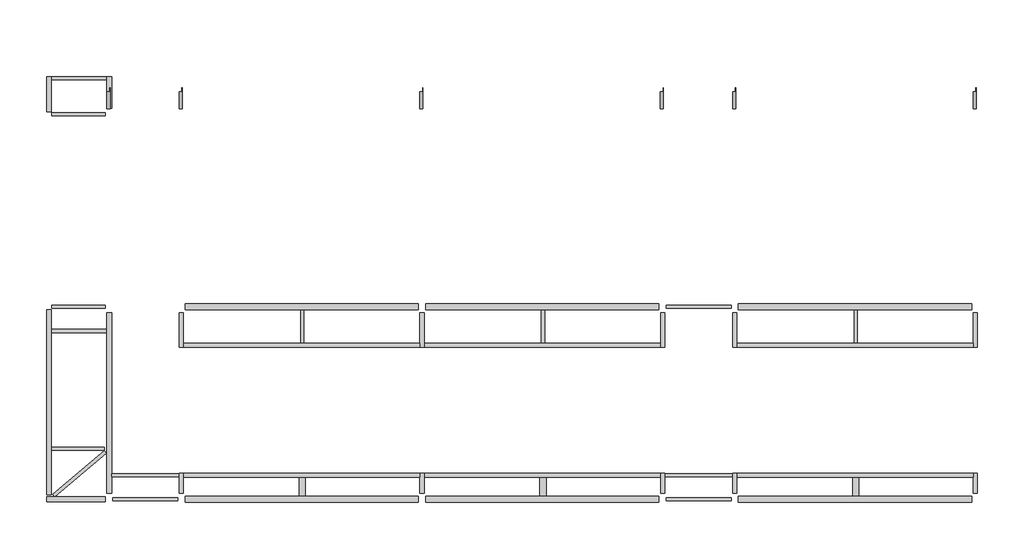
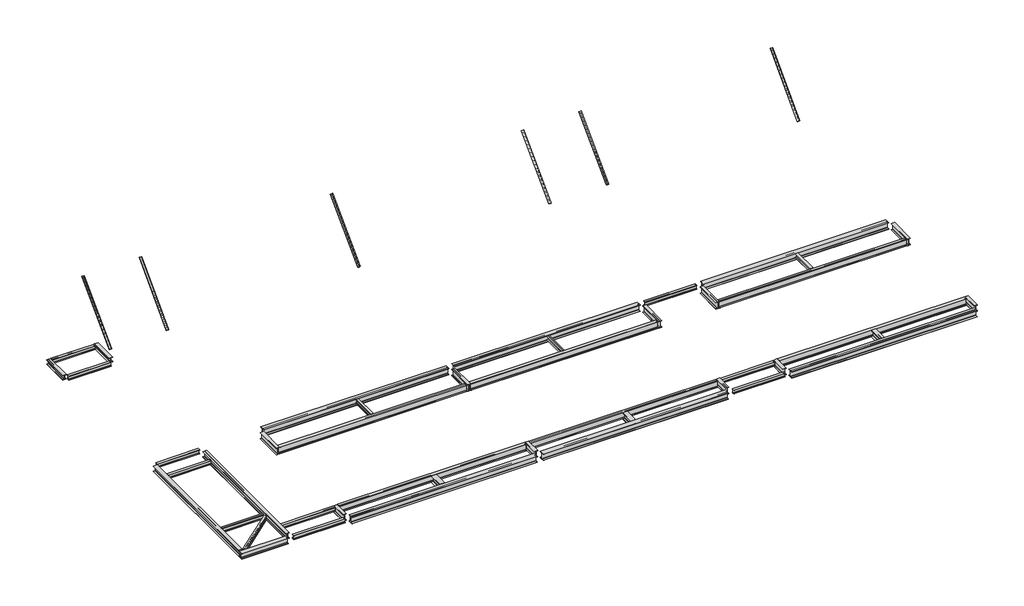
# One storey: 50 beams.
"""IFC4 building model written with IfcOpenShell, lengths in millimetres."""

import ifcopenshell
import ifcopenshell.guid

model = None  # the IFC model being written
_history = None  # IfcOwnerHistory: only IFC2X3 demands one
_inside = {}  # id of a spatial element -> (the spatial element, [elements in it])
_under = {}  # id of a project, library or spatial element -> (it, [spatial elements below it])
_declared = {}  # id of a project -> (the project, [libraries it declares])
_typed = {}  # id of a type object -> (the type object, [elements of that type])
_made_of = {}  # id of a material, layer set ... -> (it, [elements and type objects made of it])


def new_model(schema):
    """Start an empty IFC model of exactly this schema.

    Asked for "IFC4X3", IfcOpenShell would pick the latest addendum, in which some entities
    have other attributes; the version numbers below select the first issue.
    IFC2X3 requires an IfcOwnerHistory on every rooted entity: one is made here for all.
    """
    global model, _history
    if schema == "IFC4X3":
        model = ifcopenshell.file(schema_version=(4, 3, 0, 0))
    else:
        model = ifcopenshell.file(schema=schema)
    _inside.clear()
    _under.clear()
    _declared.clear()
    _typed.clear()
    _made_of.clear()
    _history = None
    if model.schema == "IFC2X3":
        org = make("IfcOrganization", Name="unknown")
        user = make(
            "IfcPersonAndOrganization",
            ThePerson=make("IfcPerson", FamilyName="unknown"),
            TheOrganization=org,
        )
        app = make(
            "IfcApplication",
            ApplicationDeveloper=org,
            Version="unknown",
            ApplicationFullName="unknown",
            ApplicationIdentifier="unknown",
        )
        _history = make(
            "IfcOwnerHistory",
            OwningUser=user,
            OwningApplication=app,
            ChangeAction="ADDED",
            CreationDate=0,
        )
    return model


def make(cls, **values):
    """One entity of the class cls with the attributes given. An attribute that is None is left unset."""
    return model.create_entity(
        cls, **{name: value for name, value in values.items() if value is not None}
    )


def rooted(cls, **values):
    """An entity with a GlobalId (a new one), such as an element, a storey or a relation."""
    return make(cls, GlobalId=ifcopenshell.guid.new(), OwnerHistory=_history, **values)


def si_unit(unit_type, name, prefix=None):
    """IfcSIUnit, for example si_unit("LENGTHUNIT", "METRE", prefix="MILLI")."""
    return make("IfcSIUnit", UnitType=unit_type, Prefix=prefix, Name=name)


def assignment(units):
    """IfcUnitAssignment: the units of a project."""
    return None if units is None else make("IfcUnitAssignment", Units=units)


def point(xyz):
    """IfcCartesianPoint."""
    return None if xyz is None else make("IfcCartesianPoint", Coordinates=xyz)


def direction(xyz):
    """IfcDirection."""
    return None if xyz is None else make("IfcDirection", DirectionRatios=xyz)


def frame(location, z_axis=None, x_axis=None):
    """IfcAxis2Placement3D, a coordinate frame: its origin and axes. An axis left out is left unset."""
    return make(
        "IfcAxis2Placement3D",
        Location=point(location),
        Axis=direction(z_axis),
        RefDirection=direction(x_axis),
    )


def frame_2d(location, x_axis=None):
    """IfcAxis2Placement2D, a coordinate frame in the plane: its origin and x axis."""
    return make(
        "IfcAxis2Placement2D", Location=point(location), RefDirection=direction(x_axis)
    )


def origin():
    """The frame at (0, 0, 0) with its axes left unset."""
    return frame((0.0, 0.0, 0.0))


def place(relative_to, where):
    """IfcLocalPlacement: puts the frame where relative to a parent placement (None: the world)."""
    return make(
        "IfcLocalPlacement", PlacementRelTo=relative_to, RelativePlacement=where
    )


def context(
    kind, dimensions, precision=None, world=None, true_north=None, identifier=None
):
    """IfcGeometricRepresentationContext, for example the 3D "Model" context."""
    return make(
        "IfcGeometricRepresentationContext",
        ContextIdentifier=identifier,
        ContextType=kind,
        CoordinateSpaceDimension=dimensions,
        Precision=precision,
        WorldCoordinateSystem=world,
        TrueNorth=true_north,
    )


def project(units=None, contexts=None):
    """IfcProject with its units and contexts."""
    return rooted(
        "IfcProject",
        Name="project",
        RepresentationContexts=contexts,
        UnitsInContext=assignment(units),
    )


def spatial(cls, under=None, at=None, **own):
    """A site, building, storey or space (cls), placed at a placement, below another one or the project."""
    s = rooted(cls, ObjectPlacement=at, **own)
    if under is not None:
        _under.setdefault(under.id(), (under, []))[1].append(s)
    return s


def polyline(points):
    """IfcPolyline through the points."""
    return make("IfcPolyline", Points=[point(p) for p in points])


def circle_curve(where, radius):
    """IfcCircle in the frame where."""
    return make("IfcCircle", Position=where, Radius=radius)


def trimmed(basis, trim1, trim2, sense, master):
    """IfcTrimmedCurve: the piece of a basis curve between two trims."""
    return make(
        "IfcTrimmedCurve",
        BasisCurve=basis,
        Trim1=trim1,
        Trim2=trim2,
        SenseAgreement=sense,
        MasterRepresentation=master,
    )


def segment(curve, same_sense, transition):
    """IfcCompositeCurveSegment."""
    return make(
        "IfcCompositeCurveSegment",
        Transition=transition,
        SameSense=same_sense,
        ParentCurve=curve,
    )


def composite_curve(segments, self_intersect=None):
    """IfcCompositeCurve: segments joined end to end."""
    return make("IfcCompositeCurve", Segments=segments, SelfIntersect=self_intersect)


def outline(outer, holes=None, kind="AREA"):
    """IfcArbitraryClosedProfileDef: a profile drawn as a closed curve; with holes, ...WithVoids."""
    if holes is None:
        return make("IfcArbitraryClosedProfileDef", ProfileType=kind, OuterCurve=outer)
    return make(
        "IfcArbitraryProfileDefWithVoids",
        ProfileType=kind,
        OuterCurve=outer,
        InnerCurves=holes,
    )


def extrude(swept, where, along, depth):
    """IfcExtrudedAreaSolid: the profile swept, set in the frame where, extruded along a direction by depth."""
    return make(
        "IfcExtrudedAreaSolid",
        SweptArea=swept,
        Position=where,
        ExtrudedDirection=direction(along),
        Depth=depth,
    )


def shape(context_of_items, identifier, shape_type, items):
    """IfcShapeRepresentation: the items that make up one representation, for example the "Body"."""
    return make(
        "IfcShapeRepresentation",
        ContextOfItems=context_of_items,
        RepresentationIdentifier=identifier,
        RepresentationType=shape_type,
        Items=items,
    )


def source(mapping_origin, context_of_items, identifier, shape_type, items):
    """IfcRepresentationMap: a shape defined once, which mapped items show again and again."""
    return make(
        "IfcRepresentationMap",
        MappingOrigin=mapping_origin,
        MappedRepresentation=shape(context_of_items, identifier, shape_type, items),
    )


def transform(
    local_origin,
    x_axis=None,
    y_axis=None,
    z_axis=None,
    scale=None,
    scale2=None,
    scale3=None,
    uniform=True,
):
    """IfcCartesianTransformationOperator3D, or its non-uniform kind. x_axis, y_axis, z_axis: its Axis1, 2, 3."""
    if uniform:
        return make(
            "IfcCartesianTransformationOperator3D",
            Axis1=direction(x_axis),
            Axis2=direction(y_axis),
            LocalOrigin=point(local_origin),
            Scale=scale,
            Axis3=direction(z_axis),
        )
    return make(
        "IfcCartesianTransformationOperator3DnonUniform",
        Axis1=direction(x_axis),
        Axis2=direction(y_axis),
        LocalOrigin=point(local_origin),
        Scale=scale,
        Axis3=direction(z_axis),
        Scale2=scale2,
        Scale3=scale3,
    )


def mapped(mapping_source, mapping_target):
    """IfcMappedItem: shows the shape of a source again, moved by a transform."""
    return make(
        "IfcMappedItem", MappingSource=mapping_source, MappingTarget=mapping_target
    )


def made_of(thing, what):
    """Note that an element or type object is made of a material, layer set ...; save() writes the relation."""
    if what is not None:
        _made_of.setdefault(what.id(), (what, []))[1].append(thing)
    return thing


def element(
    cls,
    number,
    at=None,
    inside=None,
    cuts=None,
    type_object=None,
    material=None,
    context=None,
    identifier="Body",
    shape_type=None,
    held_by="IfcProductDefinitionShape",
    body=None,
    shapes=None,
    **own,
):
    """One element of the class cls, such as IfcWall. Its Tag is "e" and its number.

    at: its placement. inside: the storey or other place that contains it. cuts: it is an
    opening in that element (IfcRelVoidsElement). A single representation is given by context,
    identifier, shape_type and body (its items); several are given by shapes. held_by: the class
    of the entity that holds the representations. save() writes the other relations.
    """
    e = rooted(cls, Tag="e%d" % number, ObjectPlacement=at, **own)
    if body is not None:
        shapes = [shape(context, identifier, shape_type, body)]
    if shapes is not None:
        e.Representation = make(held_by, Representations=shapes)
    if inside is not None:
        _inside.setdefault(inside.id(), (inside, []))[1].append(e)
    if cuts is not None:
        rooted(
            "IfcRelVoidsElement", RelatingBuildingElement=cuts, RelatedOpeningElement=e
        )
    if type_object is not None:
        _typed.setdefault(type_object.id(), (type_object, []))[1].append(e)
    return made_of(e, material)


def aggregate(whole, parts):
    """IfcRelAggregates: a whole, such as a stair, and the parts it consists of."""
    return rooted("IfcRelAggregates", RelatingObject=whole, RelatedObjects=parts)


def save(model, path):
    """Write the relations noted so far, then the file.

    IfcRelAggregates (storeys below a building ...), IfcRelContainedInSpatialStructure (elements
    in a storey), IfcRelDefinesByType, IfcRelAssociatesMaterial and IfcRelDeclares: one each for
    every whole, place, type object, material and project.
    """
    for whole, parts in _under.values():
        aggregate(whole, parts)
    for where, things in _inside.values():
        rooted(
            "IfcRelContainedInSpatialStructure",
            RelatedElements=things,
            RelatingStructure=where,
        )
    for kind, things in _typed.values():
        rooted("IfcRelDefinesByType", RelatedObjects=things, RelatingType=kind)
    for what, things in _made_of.values():
        rooted("IfcRelAssociatesMaterial", RelatedObjects=things, RelatingMaterial=what)
    for by, libraries in _declared.values():
        rooted("IfcRelDeclares", RelatingContext=by, RelatedDefinitions=libraries)
    model.write(path)


def beam_14297e1c(model_context):
    return source(origin(), model_context, "Body", "SweptSolid", [
        extrude(outline(composite_curve([segment(polyline([(36.4, 36.4), (36.4, -93.6)]), True, "CONTINUOUS"), segment(trimmed(circle_curve(frame_2d((36.4, -81.6)), 12.0), [point((36.4, -93.6))], [point((24.4, -81.6))], False, "CARTESIAN"), True, "CONTINUOUS"), segment(polyline([(24.4, -81.6), (24.4, 12.4)]), True, "CONTINUOUS"), segment(trimmed(circle_curve(frame_2d((12.4, 12.4)), 12.0), [point((24.4, 12.4))], [point((12.4, 24.4))], True, "CARTESIAN"), True, "CONTINUOUS"), segment(polyline([(12.4, 24.4), (-81.6, 24.4)]), True, "CONTINUOUS"), segment(trimmed(circle_curve(frame_2d((-81.6, 36.4)), 12.0), [point((-81.6, 24.4))], [point((-93.6, 36.4))], False, "CARTESIAN"), True, "CONTINUOUS"), segment(polyline([(-93.6, 36.4), (36.4, 36.4)]), True, "CONTINUOUS")], self_intersect=False)), frame((-1819.863551, 0.0, 0.0), z_axis=(1.0, 0.0, 0.0), x_axis=(0.0, 1.0, 0.0)), (0.0, 0.0, 1.0), 3551.9244278),
    ])


def steel_framing_w_astm_a6m_f33feb28(model_context):
    return source(origin(), model_context, "Body", "SweptSolid", [
        extrude(outline(composite_curve([segment(polyline([(67.0, -94.8), (67.0, -105.0), (-67.0, -105.0), (-67.0, -94.8), (-10.775, -94.8)]), True, "CONTINUOUS"), segment(trimmed(circle_curve(frame_2d((-10.775, -87.2)), 7.6), [point((-10.775, -94.8))], [point((-3.175, -87.2))], True, "CARTESIAN"), True, "CONTINUOUS"), segment(polyline([(-3.175, -87.2), (-3.175, 87.2)]), True, "CONTINUOUS"), segment(trimmed(circle_curve(frame_2d((-10.775, 87.2)), 7.6), [point((-3.175, 87.2))], [point((-10.775, 94.8))], True, "CARTESIAN"), True, "CONTINUOUS"), segment(polyline([(-10.775, 94.8), (-67.0, 94.8), (-67.0, 105.0), (67.0, 105.0), (67.0, 94.8), (10.775, 94.8)]), True, "CONTINUOUS"), segment(trimmed(circle_curve(frame_2d((10.775, 87.2)), 7.6), [point((10.775, 94.8))], [point((3.175, 87.2))], True, "CARTESIAN"), True, "CONTINUOUS"), segment(polyline([(3.175, 87.2), (3.175, -87.2)]), True, "CONTINUOUS"), segment(trimmed(circle_curve(frame_2d((10.775, -87.2)), 7.6), [point((3.175, -87.2))], [point((10.775, -94.8))], True, "CARTESIAN"), True, "CONTINUOUS"), segment(polyline([(10.775, -94.8), (67.0, -94.8)]), True, "CONTINUOUS")], self_intersect=False)), frame((-1346.3, 0.0, 0.0), z_axis=(1.0, 0.0, 0.0), x_axis=(0.0, 1.0, 0.0)), (0.0, 0.0, 1.0), 2692.6),
    ])


def steel_framing_w_astm_a6m_9ad7bea0(model_context):
    return source(origin(), model_context, "Body", "SweptSolid", [
        extrude(outline(composite_curve([segment(polyline([(67.0, -94.8), (67.0, -105.0), (-67.0, -105.0), (-67.0, -94.8), (-10.775, -94.8)]), True, "CONTINUOUS"), segment(trimmed(circle_curve(frame_2d((-10.775, -87.2)), 7.6), [point((-10.775, -94.8))], [point((-3.175, -87.2))], True, "CARTESIAN"), True, "CONTINUOUS"), segment(polyline([(-3.175, -87.2), (-3.175, 87.2)]), True, "CONTINUOUS"), segment(trimmed(circle_curve(frame_2d((-10.775, 87.2)), 7.6), [point((-3.175, 87.2))], [point((-10.775, 94.8))], True, "CARTESIAN"), True, "CONTINUOUS"), segment(polyline([(-10.775, 94.8), (-67.0, 94.8), (-67.0, 105.0), (67.0, 105.0), (67.0, 94.8), (10.775, 94.8)]), True, "CONTINUOUS"), segment(trimmed(circle_curve(frame_2d((10.775, 87.2)), 7.6), [point((10.775, 94.8))], [point((3.175, 87.2))], True, "CARTESIAN"), True, "CONTINUOUS"), segment(polyline([(3.175, 87.2), (3.175, -87.2)]), True, "CONTINUOUS"), segment(trimmed(circle_curve(frame_2d((10.775, -87.2)), 7.6), [point((3.175, -87.2))], [point((10.775, -94.8))], True, "CARTESIAN"), True, "CONTINUOUS"), segment(polyline([(10.775, -94.8), (67.0, -94.8)]), True, "CONTINUOUS")], self_intersect=False)), frame((-1135.3, 0.0, 0.0), z_axis=(1.0, 0.0, 0.0), x_axis=(0.0, 1.0, 0.0)), (0.0, 0.0, 1.0), 2231.6),
    ])


def steel_framing_w_astm_a6m_5f95f2a9(model_context):
    return source(origin(), model_context, "Body", "SweptSolid", [
        extrude(outline(composite_curve([segment(polyline([(67.0, -94.8), (67.0, -105.0), (-67.0, -105.0), (-67.0, -94.8), (-10.775, -94.8)]), True, "CONTINUOUS"), segment(trimmed(circle_curve(frame_2d((-10.775, -87.2)), 7.6), [point((-10.775, -94.8))], [point((-3.175, -87.2))], True, "CARTESIAN"), True, "CONTINUOUS"), segment(polyline([(-3.175, -87.2), (-3.175, 87.2)]), True, "CONTINUOUS"), segment(trimmed(circle_curve(frame_2d((-10.775, 87.2)), 7.6), [point((-3.175, 87.2))], [point((-10.775, 94.8))], True, "CARTESIAN"), True, "CONTINUOUS"), segment(polyline([(-10.775, 94.8), (-67.0, 94.8), (-67.0, 105.0), (67.0, 105.0), (67.0, 94.8), (10.775, 94.8)]), True, "CONTINUOUS"), segment(trimmed(circle_curve(frame_2d((10.775, 87.2)), 7.6), [point((10.775, 94.8))], [point((3.175, 87.2))], True, "CARTESIAN"), True, "CONTINUOUS"), segment(polyline([(3.175, 87.2), (3.175, -87.2)]), True, "CONTINUOUS"), segment(trimmed(circle_curve(frame_2d((10.775, -87.2)), 7.6), [point((3.175, -87.2))], [point((10.775, -94.8))], True, "CARTESIAN"), True, "CONTINUOUS"), segment(polyline([(10.775, -94.8), (67.0, -94.8)]), True, "CONTINUOUS")], self_intersect=False)), frame((-1401.8, 0.0, 0.0), z_axis=(1.0, 0.0, 0.0), x_axis=(0.0, 1.0, 0.0)), (0.0, 0.0, 1.0), 2803.6),
    ])


def steel_framing_w_astm_a6m_17837fc5(model_context):
    return source(origin(), model_context, "Body", "SweptSolid", [
        extrude(outline(composite_curve([segment(polyline([(127.0, -160.1), (127.0, -176.5), (-127.0, -176.5), (-127.0, -160.1), (-19.865, -160.1)]), True, "CONTINUOUS"), segment(trimmed(circle_curve(frame_2d((-19.865, -145.0)), 15.1), [point((-19.865, -160.1))], [point((-4.765, -145.0))], True, "CARTESIAN"), True, "CONTINUOUS"), segment(polyline([(-4.765, -145.0), (-4.765, 145.0)]), True, "CONTINUOUS"), segment(trimmed(circle_curve(frame_2d((-19.865, 145.0)), 15.1), [point((-4.765, 145.0))], [point((-19.865, 160.1))], True, "CARTESIAN"), True, "CONTINUOUS"), segment(polyline([(-19.865, 160.1), (-127.0, 160.1), (-127.0, 176.5), (127.0, 176.5), (127.0, 160.1), (19.865, 160.1)]), True, "CONTINUOUS"), segment(trimmed(circle_curve(frame_2d((19.865, 145.0)), 15.1), [point((19.865, 160.1))], [point((4.765, 145.0))], True, "CARTESIAN"), True, "CONTINUOUS"), segment(polyline([(4.765, 145.0), (4.765, -145.0)]), True, "CONTINUOUS"), segment(trimmed(circle_curve(frame_2d((19.865, -145.0)), 15.1), [point((4.765, -145.0))], [point((19.865, -160.1))], True, "CARTESIAN"), True, "CONTINUOUS"), segment(polyline([(19.865, -160.1), (127.0, -160.1)]), True, "CONTINUOUS")], self_intersect=False)), frame((-4846.3, 0.0, 0.0), z_axis=(1.0, 0.0, 0.0), x_axis=(0.0, 1.0, 0.0)), (0.0, 0.0, 1.0), 9692.6),
    ])


def steel_framing_w_astm_a6m_8cea9429(model_context):
    return source(origin(), model_context, "Body", "SweptSolid", [
        extrude(outline(composite_curve([segment(polyline([(101.5, -137.9), (101.5, -151.0), (-101.5, -151.0), (-101.5, -137.9), (-16.545, -137.9)]), True, "CONTINUOUS"), segment(trimmed(circle_curve(frame_2d((-16.545, -125.1)), 12.8), [point((-16.545, -137.9))], [point((-3.745, -125.1))], True, "CARTESIAN"), True, "CONTINUOUS"), segment(polyline([(-3.745, -125.1), (-3.745, 125.1)]), True, "CONTINUOUS"), segment(trimmed(circle_curve(frame_2d((-16.545, 125.1)), 12.8), [point((-3.745, 125.1))], [point((-16.545, 137.9))], True, "CARTESIAN"), True, "CONTINUOUS"), segment(polyline([(-16.545, 137.9), (-101.5, 137.9), (-101.5, 151.0), (101.5, 151.0), (101.5, 137.9), (16.545, 137.9)]), True, "CONTINUOUS"), segment(trimmed(circle_curve(frame_2d((16.545, 125.1)), 12.8), [point((16.545, 137.9))], [point((3.745, 125.1))], True, "CARTESIAN"), True, "CONTINUOUS"), segment(polyline([(3.745, 125.1), (3.745, -125.1)]), True, "CONTINUOUS"), segment(trimmed(circle_curve(frame_2d((16.545, -125.1)), 12.8), [point((3.745, -125.1))], [point((16.545, -137.9))], True, "CARTESIAN"), True, "CONTINUOUS"), segment(polyline([(16.545, -137.9), (101.5, -137.9)]), True, "CONTINUOUS")], self_intersect=False)), frame((-3753.8, 0.0, 0.0), z_axis=(1.0, 0.0, 0.0), x_axis=(0.0, 1.0, 0.0)), (0.0, 0.0, 1.0), 7507.6),
    ])


def steel_framing_w_astm_a6m_ee6b765e(model_context):
    return source(origin(), model_context, "Body", "SweptSolid", [
        extrude(outline(composite_curve([segment(polyline([(101.0, -112.5), (101.0, -123.5), (-101.0, -123.5), (-101.0, -112.5), (-16.385, -112.5)]), True, "CONTINUOUS"), segment(trimmed(circle_curve(frame_2d((-16.385, -99.8)), 12.7), [point((-16.385, -112.5))], [point((-3.685, -99.8))], True, "CARTESIAN"), True, "CONTINUOUS"), segment(polyline([(-3.685, -99.8), (-3.685, 99.8)]), True, "CONTINUOUS"), segment(trimmed(circle_curve(frame_2d((-16.385, 99.8)), 12.7), [point((-3.685, 99.8))], [point((-16.385, 112.5))], True, "CARTESIAN"), True, "CONTINUOUS"), segment(polyline([(-16.385, 112.5), (-101.0, 112.5), (-101.0, 123.5), (101.0, 123.5), (101.0, 112.5), (16.385, 112.5)]), True, "CONTINUOUS"), segment(trimmed(circle_curve(frame_2d((16.385, 99.8)), 12.7), [point((16.385, 112.5))], [point((3.685, 99.8))], True, "CARTESIAN"), True, "CONTINUOUS"), segment(polyline([(3.685, 99.8), (3.685, -99.8)]), True, "CONTINUOUS"), segment(trimmed(circle_curve(frame_2d((16.385, -99.8)), 12.7), [point((3.685, -99.8))], [point((16.385, -112.5))], True, "CARTESIAN"), True, "CONTINUOUS"), segment(polyline([(16.385, -112.5), (101.0, -112.5)]), True, "CONTINUOUS")], self_intersect=False)), frame((-634.3, 0.0, 0.0), z_axis=(1.0, 0.0, 0.0), x_axis=(0.0, 1.0, 0.0)), (0.0, 0.0, 1.0), 1451.3),
    ])


def steel_framing_w_astm_a6m_8355ed91(model_context):
    return source(origin(), model_context, "Body", "SweptSolid", [
        extrude(outline(composite_curve([segment(polyline([(67.0, -94.8), (67.0, -105.0), (-67.0, -105.0), (-67.0, -94.8), (-10.775, -94.8)]), True, "CONTINUOUS"), segment(trimmed(circle_curve(frame_2d((-10.775, -87.2)), 7.6), [point((-10.775, -94.8))], [point((-3.175, -87.2))], True, "CARTESIAN"), True, "CONTINUOUS"), segment(polyline([(-3.175, -87.2), (-3.175, 87.2)]), True, "CONTINUOUS"), segment(trimmed(circle_curve(frame_2d((-10.775, 87.2)), 7.6), [point((-3.175, 87.2))], [point((-10.775, 94.8))], True, "CARTESIAN"), True, "CONTINUOUS"), segment(polyline([(-10.775, 94.8), (-67.0, 94.8), (-67.0, 105.0), (67.0, 105.0), (67.0, 94.8), (10.775, 94.8)]), True, "CONTINUOUS"), segment(trimmed(circle_curve(frame_2d((10.775, 87.2)), 7.6), [point((10.775, 94.8))], [point((3.175, 87.2))], True, "CARTESIAN"), True, "CONTINUOUS"), segment(polyline([(3.175, 87.2), (3.175, -87.2)]), True, "CONTINUOUS"), segment(trimmed(circle_curve(frame_2d((10.775, -87.2)), 7.6), [point((3.175, -87.2))], [point((10.775, -94.8))], True, "CARTESIAN"), True, "CONTINUOUS"), segment(polyline([(10.775, -94.8), (67.0, -94.8)]), True, "CONTINUOUS")], self_intersect=False)), frame((-1136.3, 0.0, 0.0), z_axis=(1.0, 0.0, 0.0), x_axis=(0.0, 1.0, 0.0)), (0.0, 0.0, 1.0), 2272.6),
    ])


def steel_framing_w_astm_a6m_7f0d9279(model_context):
    return source(origin(), model_context, "Body", "SweptSolid", [
        extrude(outline(composite_curve([segment(polyline([(101.0, -112.5), (101.0, -123.5), (-101.0, -123.5), (-101.0, -112.5), (-16.385, -112.5)]), True, "CONTINUOUS"), segment(trimmed(circle_curve(frame_2d((-16.385, -99.8)), 12.7), [point((-16.385, -112.5))], [point((-3.685, -99.8))], True, "CARTESIAN"), True, "CONTINUOUS"), segment(polyline([(-3.685, -99.8), (-3.685, 99.8)]), True, "CONTINUOUS"), segment(trimmed(circle_curve(frame_2d((-16.385, 99.8)), 12.7), [point((-3.685, 99.8))], [point((-16.385, 112.5))], True, "CARTESIAN"), True, "CONTINUOUS"), segment(polyline([(-16.385, 112.5), (-101.0, 112.5), (-101.0, 123.5), (101.0, 123.5), (101.0, 112.5), (16.385, 112.5)]), True, "CONTINUOUS"), segment(trimmed(circle_curve(frame_2d((16.385, 99.8)), 12.7), [point((16.385, 112.5))], [point((3.685, 99.8))], True, "CARTESIAN"), True, "CONTINUOUS"), segment(polyline([(3.685, 99.8), (3.685, -99.8)]), True, "CONTINUOUS"), segment(trimmed(circle_curve(frame_2d((16.385, -99.8)), 12.7), [point((3.685, -99.8))], [point((16.385, -112.5))], True, "CARTESIAN"), True, "CONTINUOUS"), segment(polyline([(16.385, -112.5), (101.0, -112.5)]), True, "CONTINUOUS")], self_intersect=False)), frame((-503.8, 0.0, 0.0), z_axis=(1.0, 0.0, 0.0), x_axis=(0.0, 1.0, 0.0)), (0.0, 0.0, 1.0), 1320.8),
    ])


def steel_framing_w_astm_a6m_9f313648(model_context):
    return source(origin(), model_context, "Body", "SweptSolid", [
        extrude(outline(composite_curve([segment(polyline([(67.0, -94.8), (67.0, -105.0), (-67.0, -105.0), (-67.0, -94.8), (-10.775, -94.8)]), True, "CONTINUOUS"), segment(trimmed(circle_curve(frame_2d((-10.775, -87.2)), 7.6), [point((-10.775, -94.8))], [point((-3.175, -87.2))], True, "CARTESIAN"), True, "CONTINUOUS"), segment(polyline([(-3.175, -87.2), (-3.175, 87.2)]), True, "CONTINUOUS"), segment(trimmed(circle_curve(frame_2d((-10.775, 87.2)), 7.6), [point((-3.175, 87.2))], [point((-10.775, 94.8))], True, "CARTESIAN"), True, "CONTINUOUS"), segment(polyline([(-10.775, 94.8), (-67.0, 94.8), (-67.0, 105.0), (67.0, 105.0), (67.0, 94.8), (10.775, 94.8)]), True, "CONTINUOUS"), segment(trimmed(circle_curve(frame_2d((10.775, 87.2)), 7.6), [point((10.775, 94.8))], [point((3.175, 87.2))], True, "CARTESIAN"), True, "CONTINUOUS"), segment(polyline([(3.175, 87.2), (3.175, -87.2)]), True, "CONTINUOUS"), segment(trimmed(circle_curve(frame_2d((10.775, -87.2)), 7.6), [point((3.175, -87.2))], [point((10.775, -94.8))], True, "CARTESIAN"), True, "CONTINUOUS"), segment(polyline([(10.775, -94.8), (67.0, -94.8)]), True, "CONTINUOUS")], self_intersect=False)), frame((-1135.8, 0.0, 0.0), z_axis=(1.0, 0.0, 0.0), x_axis=(0.0, 1.0, 0.0)), (0.0, 0.0, 1.0), 2271.6),
    ])


def steel_framing_w_astm_a6m_8815720a(model_context):
    return source(origin(), model_context, "Body", "SweptSolid", [
        extrude(outline(composite_curve([segment(polyline([(101.5, -137.9), (101.5, -151.0), (-101.5, -151.0), (-101.5, -137.9), (-16.545, -137.9)]), True, "CONTINUOUS"), segment(trimmed(circle_curve(frame_2d((-16.545, -125.1)), 12.8), [point((-16.545, -137.9))], [point((-3.745, -125.1))], True, "CARTESIAN"), True, "CONTINUOUS"), segment(polyline([(-3.745, -125.1), (-3.745, 125.1)]), True, "CONTINUOUS"), segment(trimmed(circle_curve(frame_2d((-16.545, 125.1)), 12.8), [point((-3.745, 125.1))], [point((-16.545, 137.9))], True, "CARTESIAN"), True, "CONTINUOUS"), segment(polyline([(-16.545, 137.9), (-101.5, 137.9), (-101.5, 151.0), (101.5, 151.0), (101.5, 137.9), (16.545, 137.9)]), True, "CONTINUOUS"), segment(trimmed(circle_curve(frame_2d((16.545, 125.1)), 12.8), [point((16.545, 137.9))], [point((3.745, 125.1))], True, "CARTESIAN"), True, "CONTINUOUS"), segment(polyline([(3.745, 125.1), (3.745, -125.1)]), True, "CONTINUOUS"), segment(trimmed(circle_curve(frame_2d((16.545, -125.1)), 12.8), [point((3.745, -125.1))], [point((16.545, -137.9))], True, "CARTESIAN"), True, "CONTINUOUS"), segment(polyline([(16.545, -137.9), (101.5, -137.9)]), True, "CONTINUOUS")], self_intersect=False)), frame((-1096.3, 0.0, 0.0), z_axis=(1.0, 0.0, 0.0), x_axis=(0.0, 1.0, 0.0)), (0.0, 0.0, 1.0), 2447.8),
    ])


def steel_framing_w_astm_a6m_1b426b15(model_context):
    return source(origin(), model_context, "Body", "SweptSolid", [
        extrude(outline(composite_curve([segment(polyline([(67.0, -94.8), (67.0, -105.0), (-67.0, -105.0), (-67.0, -94.8), (-10.775, -94.8)]), True, "CONTINUOUS"), segment(trimmed(circle_curve(frame_2d((-10.775, -87.2)), 7.6), [point((-10.775, -94.8))], [point((-3.175, -87.2))], True, "CARTESIAN"), True, "CONTINUOUS"), segment(polyline([(-3.175, -87.2), (-3.175, 87.2)]), True, "CONTINUOUS"), segment(trimmed(circle_curve(frame_2d((-10.775, 87.2)), 7.6), [point((-3.175, 87.2))], [point((-10.775, 94.8))], True, "CARTESIAN"), True, "CONTINUOUS"), segment(polyline([(-10.775, 94.8), (-67.0, 94.8), (-67.0, 105.0), (67.0, 105.0), (67.0, 94.8), (10.775, 94.8)]), True, "CONTINUOUS"), segment(trimmed(circle_curve(frame_2d((10.775, 87.2)), 7.6), [point((10.775, 94.8))], [point((3.175, 87.2))], True, "CARTESIAN"), True, "CONTINUOUS"), segment(polyline([(3.175, 87.2), (3.175, -87.2)]), True, "CONTINUOUS"), segment(trimmed(circle_curve(frame_2d((10.775, -87.2)), 7.6), [point((3.175, -87.2))], [point((10.775, -94.8))], True, "CARTESIAN"), True, "CONTINUOUS"), segment(polyline([(10.775, -94.8), (67.0, -94.8)]), True, "CONTINUOUS")], self_intersect=False)), frame((-1135.8, 0.0, 0.0), z_axis=(1.0, 0.0, 0.0), x_axis=(0.0, 1.0, 0.0)), (0.0, 0.0, 1.0), 2189.1),
    ])


def steel_framing_w_astm_a6m_97b597d5(model_context):
    return source(origin(), model_context, "Body", "SweptSolid", [
        extrude(outline(composite_curve([segment(polyline([(101.5, -137.9), (101.5, -151.0), (-101.5, -151.0), (-101.5, -137.9), (-16.545, -137.9)]), True, "CONTINUOUS"), segment(trimmed(circle_curve(frame_2d((-16.545, -125.1)), 12.8), [point((-16.545, -137.9))], [point((-3.745, -125.1))], True, "CARTESIAN"), True, "CONTINUOUS"), segment(polyline([(-3.745, -125.1), (-3.745, 125.1)]), True, "CONTINUOUS"), segment(trimmed(circle_curve(frame_2d((-16.545, 125.1)), 12.8), [point((-3.745, 125.1))], [point((-16.545, 137.9))], True, "CARTESIAN"), True, "CONTINUOUS"), segment(polyline([(-16.545, 137.9), (-101.5, 137.9), (-101.5, 151.0), (101.5, 151.0), (101.5, 137.9), (16.545, 137.9)]), True, "CONTINUOUS"), segment(trimmed(circle_curve(frame_2d((16.545, 125.1)), 12.8), [point((16.545, 137.9))], [point((3.745, 125.1))], True, "CARTESIAN"), True, "CONTINUOUS"), segment(polyline([(3.745, 125.1), (3.745, -125.1)]), True, "CONTINUOUS"), segment(trimmed(circle_curve(frame_2d((16.545, -125.1)), 12.8), [point((3.745, -125.1))], [point((16.545, -137.9))], True, "CARTESIAN"), True, "CONTINUOUS"), segment(polyline([(16.545, -137.9), (101.5, -137.9)]), True, "CONTINUOUS")], self_intersect=False)), frame((-3884.3, 0.0, 0.0), z_axis=(1.0, 0.0, 0.0), x_axis=(0.0, 1.0, 0.0)), (0.0, 0.0, 1.0), 7698.8),
    ])


def steel_framing_w_astm_a6m_8d3d16c6(model_context):
    return source(origin(), model_context, "Body", "SweptSolid", [
        extrude(outline(composite_curve([segment(polyline([(67.0, -94.8), (67.0, -105.0), (-67.0, -105.0), (-67.0, -94.8), (-10.775, -94.8)]), True, "CONTINUOUS"), segment(trimmed(circle_curve(frame_2d((-10.775, -87.2)), 7.6), [point((-10.775, -94.8))], [point((-3.175, -87.2))], True, "CARTESIAN"), True, "CONTINUOUS"), segment(polyline([(-3.175, -87.2), (-3.175, 87.2)]), True, "CONTINUOUS"), segment(trimmed(circle_curve(frame_2d((-10.775, 87.2)), 7.6), [point((-3.175, 87.2))], [point((-10.775, 94.8))], True, "CARTESIAN"), True, "CONTINUOUS"), segment(polyline([(-10.775, 94.8), (-67.0, 94.8), (-67.0, 105.0), (67.0, 105.0), (67.0, 94.8), (10.775, 94.8)]), True, "CONTINUOUS"), segment(trimmed(circle_curve(frame_2d((10.775, 87.2)), 7.6), [point((10.775, 94.8))], [point((3.175, 87.2))], True, "CARTESIAN"), True, "CONTINUOUS"), segment(polyline([(3.175, 87.2), (3.175, -87.2)]), True, "CONTINUOUS"), segment(trimmed(circle_curve(frame_2d((10.775, -87.2)), 7.6), [point((3.175, -87.2))], [point((10.775, -94.8))], True, "CARTESIAN"), True, "CONTINUOUS"), segment(polyline([(10.775, -94.8), (67.0, -94.8)]), True, "CONTINUOUS")], self_intersect=False)), frame((-1382.2, 0.0, 0.0), z_axis=(1.0, 0.0, 0.0), x_axis=(0.0, 1.0, 0.0)), (0.0, 0.0, 1.0), 2813.1),
    ])


def steel_framing_w_astm_a6m_0a69f8b6(model_context):
    return source(origin(), model_context, "Body", "SweptSolid", [
        extrude(outline(composite_curve([segment(polyline([(67.0, -94.8), (67.0, -105.0), (-67.0, -105.0), (-67.0, -94.8), (-10.775, -94.8)]), True, "CONTINUOUS"), segment(trimmed(circle_curve(frame_2d((-10.775, -87.2)), 7.6), [point((-10.775, -94.8))], [point((-3.175, -87.2))], True, "CARTESIAN"), True, "CONTINUOUS"), segment(polyline([(-3.175, -87.2), (-3.175, 87.2)]), True, "CONTINUOUS"), segment(trimmed(circle_curve(frame_2d((-10.775, 87.2)), 7.6), [point((-3.175, 87.2))], [point((-10.775, 94.8))], True, "CARTESIAN"), True, "CONTINUOUS"), segment(polyline([(-10.775, 94.8), (-67.0, 94.8), (-67.0, 105.0), (67.0, 105.0), (67.0, 94.8), (10.775, 94.8)]), True, "CONTINUOUS"), segment(trimmed(circle_curve(frame_2d((10.775, 87.2)), 7.6), [point((10.775, 94.8))], [point((3.175, 87.2))], True, "CARTESIAN"), True, "CONTINUOUS"), segment(polyline([(3.175, 87.2), (3.175, -87.2)]), True, "CONTINUOUS"), segment(trimmed(circle_curve(frame_2d((10.775, -87.2)), 7.6), [point((3.175, -87.2))], [point((10.775, -94.8))], True, "CARTESIAN"), True, "CONTINUOUS"), segment(polyline([(10.775, -94.8), (67.0, -94.8)]), True, "CONTINUOUS")], self_intersect=False)), frame((-1385.8, 0.0, 0.0), z_axis=(1.0, 0.0, 0.0), x_axis=(0.0, 1.0, 0.0)), (0.0, 0.0, 1.0), 2787.6),
    ])


def steel_framing_w_astm_a6m_0f62209b(model_context):
    return source(origin(), model_context, "Body", "SweptSolid", [
        extrude(outline(composite_curve([segment(polyline([(85.5, -166.4), (85.5, -178.0), (-85.5, -178.0), (-85.5, -166.4), (-13.72, -166.4)]), True, "CONTINUOUS"), segment(trimmed(circle_curve(frame_2d((-13.72, -156.3)), 10.1), [point((-13.72, -166.4))], [point((-3.62, -156.3))], True, "CARTESIAN"), True, "CONTINUOUS"), segment(polyline([(-3.62, -156.3), (-3.62, 156.3)]), True, "CONTINUOUS"), segment(trimmed(circle_curve(frame_2d((-13.72, 156.3)), 10.1), [point((-3.62, 156.3))], [point((-13.72, 166.4))], True, "CARTESIAN"), True, "CONTINUOUS"), segment(polyline([(-13.72, 166.4), (-85.5, 166.4), (-85.5, 178.0), (85.5, 178.0), (85.5, 166.4), (13.72, 166.4)]), True, "CONTINUOUS"), segment(trimmed(circle_curve(frame_2d((13.72, 156.3)), 10.1), [point((13.72, 166.4))], [point((3.62, 156.3))], True, "CARTESIAN"), True, "CONTINUOUS"), segment(polyline([(3.62, 156.3), (3.62, -156.3)]), True, "CONTINUOUS"), segment(trimmed(circle_curve(frame_2d((13.72, -156.3)), 10.1), [point((3.62, -156.3))], [point((13.72, -166.4))], True, "CARTESIAN"), True, "CONTINUOUS"), segment(polyline([(13.72, -166.4), (85.5, -166.4)]), True, "CONTINUOUS")], self_intersect=False)), frame((-253.8, 0.0, 0.0), z_axis=(1.0, 0.0, 0.0), x_axis=(0.0, 1.0, 0.0)), (0.0, 0.0, 1.0), 839.3),
    ])


def steel_framing_w_astm_a6m_8e55c2dc(model_context):
    return source(origin(), model_context, "Body", "SweptSolid", [
        extrude(outline(composite_curve([segment(polyline([(85.5, -166.4), (85.5, -178.0), (-85.5, -178.0), (-85.5, -166.4), (-13.72, -166.4)]), True, "CONTINUOUS"), segment(trimmed(circle_curve(frame_2d((-13.72, -156.3)), 10.1), [point((-13.72, -166.4))], [point((-3.62, -156.3))], True, "CARTESIAN"), True, "CONTINUOUS"), segment(polyline([(-3.62, -156.3), (-3.62, 156.3)]), True, "CONTINUOUS"), segment(trimmed(circle_curve(frame_2d((-13.72, 156.3)), 10.1), [point((-3.62, 156.3))], [point((-13.72, 166.4))], True, "CARTESIAN"), True, "CONTINUOUS"), segment(polyline([(-13.72, 166.4), (-85.5, 166.4), (-85.5, 178.0), (85.5, 178.0), (85.5, 166.4), (13.72, 166.4)]), True, "CONTINUOUS"), segment(trimmed(circle_curve(frame_2d((13.72, 156.3)), 10.1), [point((13.72, 166.4))], [point((3.62, 156.3))], True, "CARTESIAN"), True, "CONTINUOUS"), segment(polyline([(3.62, 156.3), (3.62, -156.3)]), True, "CONTINUOUS"), segment(trimmed(circle_curve(frame_2d((13.72, -156.3)), 10.1), [point((3.62, -156.3))], [point((13.72, -166.4))], True, "CARTESIAN"), True, "CONTINUOUS"), segment(polyline([(13.72, -166.4), (85.5, -166.4)]), True, "CONTINUOUS")], self_intersect=False)), frame((-4901.8, 0.0, 0.0), z_axis=(1.0, 0.0, 0.0), x_axis=(0.0, 1.0, 0.0)), (0.0, 0.0, 1.0), 9803.6),
    ])


def steel_framing_w_astm_a6m_0ec37d14(model_context):
    return source(origin(), model_context, "Body", "SweptSolid", [
        extrude(outline(composite_curve([segment(polyline([(85.5, -166.4), (85.5, -178.0), (-85.5, -178.0), (-85.5, -166.4), (-13.72, -166.4)]), True, "CONTINUOUS"), segment(trimmed(circle_curve(frame_2d((-13.72, -156.3)), 10.1), [point((-13.72, -166.4))], [point((-3.62, -156.3))], True, "CARTESIAN"), True, "CONTINUOUS"), segment(polyline([(-3.62, -156.3), (-3.62, 156.3)]), True, "CONTINUOUS"), segment(trimmed(circle_curve(frame_2d((-13.72, 156.3)), 10.1), [point((-3.62, 156.3))], [point((-13.72, 166.4))], True, "CARTESIAN"), True, "CONTINUOUS"), segment(polyline([(-13.72, 166.4), (-85.5, 166.4), (-85.5, 178.0), (85.5, 178.0), (85.5, 166.4), (13.72, 166.4)]), True, "CONTINUOUS"), segment(trimmed(circle_curve(frame_2d((13.72, 156.3)), 10.1), [point((13.72, 166.4))], [point((3.62, 156.3))], True, "CARTESIAN"), True, "CONTINUOUS"), segment(polyline([(3.62, 156.3), (3.62, -156.3)]), True, "CONTINUOUS"), segment(trimmed(circle_curve(frame_2d((13.72, -156.3)), 10.1), [point((3.62, -156.3))], [point((13.72, -166.4))], True, "CARTESIAN"), True, "CONTINUOUS"), segment(polyline([(13.72, -166.4), (85.5, -166.4)]), True, "CONTINUOUS")], self_intersect=False)), frame((-553.8, 0.0, 0.0), z_axis=(1.0, 0.0, 0.0), x_axis=(0.0, 1.0, 0.0)), (0.0, 0.0, 1.0), 1439.3),
    ])


def steel_framing_w_astm_a6m_e50dfa28(model_context):
    return source(origin(), model_context, "Body", "SweptSolid", [
        extrude(outline(composite_curve([segment(polyline([(67.0, -94.8), (67.0, -105.0), (-67.0, -105.0), (-67.0, -94.8), (-10.775, -94.8)]), True, "CONTINUOUS"), segment(trimmed(circle_curve(frame_2d((-10.775, -87.2)), 7.6), [point((-10.775, -94.8))], [point((-3.175, -87.2))], True, "CARTESIAN"), True, "CONTINUOUS"), segment(polyline([(-3.175, -87.2), (-3.175, 87.2)]), True, "CONTINUOUS"), segment(trimmed(circle_curve(frame_2d((-10.775, 87.2)), 7.6), [point((-3.175, 87.2))], [point((-10.775, 94.8))], True, "CARTESIAN"), True, "CONTINUOUS"), segment(polyline([(-10.775, 94.8), (-67.0, 94.8), (-67.0, 105.0), (67.0, 105.0), (67.0, 94.8), (10.775, 94.8)]), True, "CONTINUOUS"), segment(trimmed(circle_curve(frame_2d((10.775, 87.2)), 7.6), [point((10.775, 94.8))], [point((3.175, 87.2))], True, "CARTESIAN"), True, "CONTINUOUS"), segment(polyline([(3.175, 87.2), (3.175, -87.2)]), True, "CONTINUOUS"), segment(trimmed(circle_curve(frame_2d((10.775, -87.2)), 7.6), [point((3.175, -87.2))], [point((10.775, -94.8))], True, "CARTESIAN"), True, "CONTINUOUS"), segment(polyline([(10.775, -94.8), (67.0, -94.8)]), True, "CONTINUOUS")], self_intersect=False)), frame((-660.3, 0.0, 0.0), z_axis=(1.0, 0.0, 0.0), x_axis=(0.0, 1.0, 0.0)), (0.0, 0.0, 1.0), 1362.1),
    ])


def steel_framing_w_astm_a6m_e4d07942(model_context):
    return source(origin(), model_context, "Body", "SweptSolid", [
        extrude(outline(composite_curve([segment(polyline([(127.0, -160.1), (127.0, -176.5), (-127.0, -176.5), (-127.0, -160.1), (-19.865, -160.1)]), True, "CONTINUOUS"), segment(trimmed(circle_curve(frame_2d((-19.865, -145.0)), 15.1), [point((-19.865, -160.1))], [point((-4.765, -145.0))], True, "CARTESIAN"), True, "CONTINUOUS"), segment(polyline([(-4.765, -145.0), (-4.765, 145.0)]), True, "CONTINUOUS"), segment(trimmed(circle_curve(frame_2d((-19.865, 145.0)), 15.1), [point((-4.765, 145.0))], [point((-19.865, 160.1))], True, "CARTESIAN"), True, "CONTINUOUS"), segment(polyline([(-19.865, 160.1), (-127.0, 160.1), (-127.0, 176.5), (127.0, 176.5), (127.0, 160.1), (19.865, 160.1)]), True, "CONTINUOUS"), segment(trimmed(circle_curve(frame_2d((19.865, 145.0)), 15.1), [point((19.865, 160.1))], [point((4.765, 145.0))], True, "CARTESIAN"), True, "CONTINUOUS"), segment(polyline([(4.765, 145.0), (4.765, -145.0)]), True, "CONTINUOUS"), segment(trimmed(circle_curve(frame_2d((19.865, -145.0)), 15.1), [point((4.765, -145.0))], [point((19.865, -160.1))], True, "CARTESIAN"), True, "CONTINUOUS"), segment(polyline([(19.865, -160.1), (127.0, -160.1)]), True, "CONTINUOUS")], self_intersect=False)), frame((-360.3, 0.0, 0.0), z_axis=(1.0, 0.0, 0.0), x_axis=(0.0, 1.0, 0.0)), (0.0, 0.0, 1.0), 762.1),
    ])


model = new_model("IFC4")

# Units and contexts
model_context = context("Model", 3, world=origin())
ifc_project = project(units=[si_unit("LENGTHUNIT", "METRE", prefix="MILLI")], contexts=[model_context])

# Site, building, storey
site = spatial("IfcSite", under=ifc_project)
building = spatial("IfcBuilding", under=site)
storey = spatial("IfcBuildingStorey", under=building, Name="T.O.S(2-1)", Elevation=519.8243501)

# Beams
placement = place(None, origin())
beam_shape = beam_14297e1c(model_context)
element("IfcBeam", 1, at=placement, inside=storey, context=model_context, shape_type="MappedRepresentation", body=[
    mapped(beam_shape, transform((0.0, 23979.0755192, 2228.3230522), x_axis=(0.0, -0.6992553162952158, -0.714872018359145), y_axis=(1.0, 0.0, 0.0), z_axis=(0.0, -0.714872018359145, 0.6992553162952158))),
])
element("IfcBeam", 2, at=placement, inside=storey, context=model_context, shape_type="MappedRepresentation", body=[
    mapped(beam_shape, transform((3000.0, 23979.0755192, 2228.3230522), x_axis=(0.0, -0.6992553162952158, -0.714872018359145), y_axis=(1.0, 0.0, 0.0), z_axis=(0.0, -0.714872018359145, 0.6992553162952158))),
])
element("IfcBeam", 3, at=placement, inside=storey, context=model_context, shape_type="MappedRepresentation", body=[
    mapped(beam_shape, transform((13000.0, 23979.0755192, 2228.3230522), x_axis=(0.0, -0.6992553162952158, -0.714872018359145), y_axis=(1.0, 0.0, 0.0), z_axis=(0.0, -0.714872018359145, 0.6992553162952158))),
])
element("IfcBeam", 4, at=placement, inside=storey, context=model_context, shape_type="MappedRepresentation", body=[
    mapped(beam_shape, transform((23000.0, 23979.0755192, 2228.3230522), x_axis=(0.0, -0.6992553162952158, -0.714872018359145), y_axis=(1.0, 0.0, 0.0), z_axis=(0.0, -0.714872018359145, 0.6992553162952158))),
])
element("IfcBeam", 5, at=placement, inside=storey, context=model_context, shape_type="MappedRepresentation", body=[
    mapped(beam_shape, transform((26000.0, 23979.0755192, 2228.3230522), x_axis=(0.0, -0.6992553162952158, -0.714872018359145), y_axis=(1.0, 0.0, 0.0), z_axis=(0.0, -0.714872018359145, 0.6992553162952158))),
])
element("IfcBeam", 6, at=placement, inside=storey, context=model_context, shape_type="MappedRepresentation", body=[
    mapped(beam_shape, transform((36000.0, 23979.0755192, 2228.3230522), x_axis=(0.0, -0.6992553162952158, -0.714872018359145), y_axis=(1.0, 0.0, 0.0), z_axis=(0.0, -0.714872018359145, 0.6992553162952158))),
])
steel_framing_w_astm_a6m_shape = steel_framing_w_astm_a6m_f33feb28(model_context)
element("IfcBeam", 7, ObjectType="Steel Framing_W_ASTM A6M", at=placement, inside=storey, context=model_context, shape_type="MappedRepresentation", body=[
    mapped(steel_framing_w_astm_a6m_shape, transform((1500.0, 6499.5208589, 414.8243501), x_axis=(1.0, 0.0, 0.0), y_axis=(0.0, 1.0, 0.0), z_axis=(0.0, 0.0, 1.0))),
])
element("IfcBeam", 8, ObjectType="Steel Framing_W_ASTM A6M", at=placement, inside=storey, context=model_context, shape_type="MappedRepresentation", body=[
    mapped(steel_framing_w_astm_a6m_shape, transform((24500.0, 6499.5208589, 414.8243501), x_axis=(1.0, 0.0, 0.0), y_axis=(0.0, 1.0, 0.0), z_axis=(0.0, 0.0, 1.0))),
])
element("IfcBeam", 9, ObjectType="Steel Framing_W_ASTM A6M", at=placement, inside=storey, context=model_context, shape_type="MappedRepresentation", body=[
    mapped(steel_framing_w_astm_a6m_shape, transform((24500.0, 14499.5208589, 414.8243501), x_axis=(1.0, 0.0, 0.0), y_axis=(0.0, 1.0, 0.0), z_axis=(0.0, 0.0, 1.0))),
])
steel_framing_w_astm_a6m_2_shape = steel_framing_w_astm_a6m_9ad7bea0(model_context)
element("IfcBeam", 10, ObjectType="Steel Framing_W_ASTM A6M", at=placement, inside=storey, context=model_context, shape_type="MappedRepresentation", body=[
    mapped(steel_framing_w_astm_a6m_2_shape, transform((-1250.0, 22499.5208589, 414.8243501), x_axis=(1.0, 0.0, 0.0), y_axis=(0.0, 1.0, 0.0), z_axis=(0.0, 0.0, 1.0))),
])
element("IfcBeam", 11, ObjectType="Steel Framing_W_ASTM A6M", at=placement, inside=storey, context=model_context, shape_type="MappedRepresentation", body=[
    mapped(steel_framing_w_astm_a6m_2_shape, transform((-1250.0, 14499.5208589, 414.8243501), x_axis=(1.0, 0.0, 0.0), y_axis=(0.0, 1.0, 0.0), z_axis=(0.0, 0.0, 1.0))),
])
steel_framing_w_astm_a6m_3_shape = steel_framing_w_astm_a6m_5f95f2a9(model_context)
element("IfcBeam", 12, ObjectType="Steel Framing_W_ASTM A6M", at=placement, inside=storey, context=model_context, shape_type="MappedRepresentation", body=[
    mapped(steel_framing_w_astm_a6m_3_shape, transform((24500.0, 7499.5208589, 414.8243501), x_axis=(1.0, 0.0, 0.0), y_axis=(0.0, 1.0, 0.0), z_axis=(0.0, 0.0, 1.0))),
])
steel_framing_w_astm_a6m_4_shape = steel_framing_w_astm_a6m_17837fc5(model_context)
element("IfcBeam", 13, ObjectType="Steel Framing_W_ASTM A6M", at=placement, inside=storey, context=model_context, shape_type="MappedRepresentation", body=[
    mapped(steel_framing_w_astm_a6m_4_shape, transform((8000.0, 6499.5208589, 343.3243501), x_axis=(1.0, 0.0, 0.0), y_axis=(0.0, 1.0, 0.0), z_axis=(0.0, 0.0, 1.0))),
])
element("IfcBeam", 14, ObjectType="Steel Framing_W_ASTM A6M", at=placement, inside=storey, context=model_context, shape_type="MappedRepresentation", body=[
    mapped(steel_framing_w_astm_a6m_4_shape, transform((18000.0, 6499.5208589, 343.3243501), x_axis=(1.0, 0.0, 0.0), y_axis=(0.0, 1.0, 0.0), z_axis=(0.0, 0.0, 1.0))),
])
element("IfcBeam", 15, ObjectType="Steel Framing_W_ASTM A6M", at=placement, inside=storey, context=model_context, shape_type="MappedRepresentation", body=[
    mapped(steel_framing_w_astm_a6m_4_shape, transform((31000.0, 6499.5208589, 343.3243501), x_axis=(1.0, 0.0, 0.0), y_axis=(0.0, 1.0, 0.0), z_axis=(0.0, 0.0, 1.0))),
])
element("IfcBeam", 16, ObjectType="Steel Framing_W_ASTM A6M", at=placement, inside=storey, context=model_context, shape_type="MappedRepresentation", body=[
    mapped(steel_framing_w_astm_a6m_4_shape, transform((8000.0, 14499.5208589, 343.3243501), x_axis=(1.0, 0.0, 0.0), y_axis=(0.0, 1.0, 0.0), z_axis=(0.0, 0.0, 1.0))),
])
element("IfcBeam", 17, ObjectType="Steel Framing_W_ASTM A6M", at=placement, inside=storey, context=model_context, shape_type="MappedRepresentation", body=[
    mapped(steel_framing_w_astm_a6m_4_shape, transform((18000.0, 14499.5208589, 343.3243501), x_axis=(1.0, 0.0, 0.0), y_axis=(0.0, 1.0, 0.0), z_axis=(0.0, 0.0, 1.0))),
])
element("IfcBeam", 18, ObjectType="Steel Framing_W_ASTM A6M", at=placement, inside=storey, context=model_context, shape_type="MappedRepresentation", body=[
    mapped(steel_framing_w_astm_a6m_4_shape, transform((31000.0, 14499.5208589, 343.3243501), x_axis=(1.0, 0.0, 0.0), y_axis=(0.0, 1.0, 0.0), z_axis=(0.0, 0.0, 1.0))),
])
steel_framing_w_astm_a6m_5_shape = steel_framing_w_astm_a6m_8cea9429(model_context)
element("IfcBeam", 19, ObjectType="Steel Framing_W_ASTM A6M", at=placement, inside=storey, context=model_context, shape_type="MappedRepresentation", body=[
    mapped(steel_framing_w_astm_a6m_5_shape, transform((0.0, 10499.5208589, 368.8243501), x_axis=(0.0, -1.0, 0.0), y_axis=(1.0, 0.0, 0.0), z_axis=(0.0, 0.0, 1.0))),
])
steel_framing_w_astm_a6m_6_shape = steel_framing_w_astm_a6m_ee6b765e(model_context)
element("IfcBeam", 20, ObjectType="Steel Framing_W_ASTM A6M", at=placement, inside=storey, context=model_context, shape_type="MappedRepresentation", body=[
    mapped(steel_framing_w_astm_a6m_6_shape, transform((-2500.0, 23249.5208589, 396.3243501), x_axis=(0.0, 1.0, 0.0), y_axis=(-1.0, 0.0, 0.0), z_axis=(0.0, 0.0, 1.0))),
])
steel_framing_w_astm_a6m_7_shape = steel_framing_w_astm_a6m_8355ed91(model_context)
element("IfcBeam", 21, ObjectType="Steel Framing_W_ASTM A6M", at=placement, inside=storey, context=model_context, shape_type="MappedRepresentation", body=[
    mapped(steel_framing_w_astm_a6m_7_shape, transform((-1250.0, 23999.5208589, 414.8243501), x_axis=(1.0, 0.0, 0.0), y_axis=(0.0, 1.0, 0.0), z_axis=(0.0, 0.0, 1.0))),
])
steel_framing_w_astm_a6m_8_shape = steel_framing_w_astm_a6m_7f0d9279(model_context)
element("IfcBeam", 22, ObjectType="Steel Framing_W_ASTM A6M", at=placement, inside=storey, context=model_context, shape_type="MappedRepresentation", body=[
    mapped(steel_framing_w_astm_a6m_8_shape, transform((0.0, 23249.5208589, 396.3243501), x_axis=(0.0, 1.0, 0.0), y_axis=(-1.0, 0.0, 0.0), z_axis=(0.0, 0.0, 1.0))),
])
steel_framing_w_astm_a6m_9_shape = steel_framing_w_astm_a6m_9f313648(model_context)
element("IfcBeam", 23, ObjectType="Steel Framing_W_ASTM A6M", at=placement, inside=storey, context=model_context, shape_type="MappedRepresentation", body=[
    mapped(steel_framing_w_astm_a6m_9_shape, transform((-1250.0, 13499.5208589, 414.8243501), x_axis=(1.0, 0.0, 0.0), y_axis=(0.0, 1.0, 0.0), z_axis=(0.0, 0.0, 1.0))),
])
steel_framing_w_astm_a6m_10_shape = steel_framing_w_astm_a6m_8815720a(model_context)
element("IfcBeam", 24, ObjectType="Steel Framing_W_ASTM A6M", at=placement, inside=storey, context=model_context, shape_type="MappedRepresentation", body=[
    mapped(steel_framing_w_astm_a6m_10_shape, transform((-1250.0, 6499.5208589, 368.8243501), x_axis=(-1.0, 0.0, 0.0), y_axis=(0.0, -1.0, 0.0), z_axis=(0.0, 0.0, 1.0))),
])
steel_framing_w_astm_a6m_11_shape = steel_framing_w_astm_a6m_1b426b15(model_context)
element("IfcBeam", 25, ObjectType="Steel Framing_W_ASTM A6M", at=placement, inside=storey, context=model_context, shape_type="MappedRepresentation", body=[
    mapped(steel_framing_w_astm_a6m_11_shape, transform((-1250.0, 8599.5208589, 414.8243501), x_axis=(1.0, 0.0, 0.0), y_axis=(0.0, 1.0, 0.0), z_axis=(0.0, 0.0, 1.0))),
])
steel_framing_w_astm_a6m_12_shape = steel_framing_w_astm_a6m_97b597d5(model_context)
element("IfcBeam", 26, ObjectType="Steel Framing_W_ASTM A6M", at=placement, inside=storey, context=model_context, shape_type="MappedRepresentation", body=[
    mapped(steel_framing_w_astm_a6m_12_shape, transform((-2500.0, 10499.5208589, 368.8243501), x_axis=(0.0, -1.0, 0.0), y_axis=(1.0, 0.0, 0.0), z_axis=(0.0, 0.0, 1.0))),
])
steel_framing_w_astm_a6m_13_shape = steel_framing_w_astm_a6m_8d3d16c6(model_context)
element("IfcBeam", 27, ObjectType="Steel Framing_W_ASTM A6M", at=placement, inside=storey, context=model_context, shape_type="MappedRepresentation", body=[
    mapped(steel_framing_w_astm_a6m_13_shape, transform((-1250.0, 7549.5208589, 414.8243501), x_axis=(0.7657048647896111, 0.6431920864232732, 0.0), y_axis=(-0.6431920864232732, 0.7657048647896111, 0.0), z_axis=(0.0, 0.0, 1.0))),
])
steel_framing_w_astm_a6m_14_shape = steel_framing_w_astm_a6m_0a69f8b6(model_context)
element("IfcBeam", 28, ObjectType="Steel Framing_W_ASTM A6M", at=placement, inside=storey, context=model_context, shape_type="MappedRepresentation", body=[
    mapped(steel_framing_w_astm_a6m_14_shape, transform((1500.0, 7499.5208589, 414.8243501), x_axis=(1.0, 0.0, 0.0), y_axis=(0.0, 1.0, 0.0), z_axis=(0.0, 0.0, 1.0))),
])
steel_framing_w_astm_a6m_15_shape = steel_framing_w_astm_a6m_0f62209b(model_context)
element("IfcBeam", 29, ObjectType="Steel Framing_W_ASTM A6M", at=placement, inside=storey, context=model_context, shape_type="MappedRepresentation", body=[
    mapped(steel_framing_w_astm_a6m_15_shape, transform((3000.0, 6999.5208589, 341.8243501), x_axis=(0.0, 1.0, 0.0), y_axis=(-1.0, 0.0, 0.0), z_axis=(0.0, 0.0, 1.0))),
])
element("IfcBeam", 30, ObjectType="Steel Framing_W_ASTM A6M", at=placement, inside=storey, context=model_context, shape_type="MappedRepresentation", body=[
    mapped(steel_framing_w_astm_a6m_15_shape, transform((13000.0, 6999.5208589, 341.8243501), x_axis=(0.0, 1.0, 0.0), y_axis=(-1.0, 0.0, 0.0), z_axis=(0.0, 0.0, 1.0))),
])
element("IfcBeam", 31, ObjectType="Steel Framing_W_ASTM A6M", at=placement, inside=storey, context=model_context, shape_type="MappedRepresentation", body=[
    mapped(steel_framing_w_astm_a6m_15_shape, transform((23000.0, 6999.5208589, 341.8243501), x_axis=(0.0, 1.0, 0.0), y_axis=(-1.0, 0.0, 0.0), z_axis=(0.0, 0.0, 1.0))),
])
element("IfcBeam", 32, ObjectType="Steel Framing_W_ASTM A6M", at=placement, inside=storey, context=model_context, shape_type="MappedRepresentation", body=[
    mapped(steel_framing_w_astm_a6m_15_shape, transform((26000.0, 6999.5208589, 341.8243501), x_axis=(0.0, 1.0, 0.0), y_axis=(-1.0, 0.0, 0.0), z_axis=(0.0, 0.0, 1.0))),
])
element("IfcBeam", 33, ObjectType="Steel Framing_W_ASTM A6M", at=placement, inside=storey, context=model_context, shape_type="MappedRepresentation", body=[
    mapped(steel_framing_w_astm_a6m_15_shape, transform((36000.0, 6999.5208589, 341.8243501), x_axis=(0.0, 1.0, 0.0), y_axis=(-1.0, 0.0, 0.0), z_axis=(0.0, 0.0, 1.0))),
])
steel_framing_w_astm_a6m_16_shape = steel_framing_w_astm_a6m_8e55c2dc(model_context)
element("IfcBeam", 34, ObjectType="Steel Framing_W_ASTM A6M", at=placement, inside=storey, context=model_context, shape_type="MappedRepresentation", body=[
    mapped(steel_framing_w_astm_a6m_16_shape, transform((8000.0, 7499.5208589, 341.8243501), x_axis=(1.0, 0.0, 0.0), y_axis=(0.0, 1.0, 0.0), z_axis=(0.0, 0.0, 1.0))),
])
element("IfcBeam", 35, ObjectType="Steel Framing_W_ASTM A6M", at=placement, inside=storey, context=model_context, shape_type="MappedRepresentation", body=[
    mapped(steel_framing_w_astm_a6m_16_shape, transform((18000.0, 7499.5208589, 341.8243501), x_axis=(1.0, 0.0, 0.0), y_axis=(0.0, 1.0, 0.0), z_axis=(0.0, 0.0, 1.0))),
])
element("IfcBeam", 36, ObjectType="Steel Framing_W_ASTM A6M", at=placement, inside=storey, context=model_context, shape_type="MappedRepresentation", body=[
    mapped(steel_framing_w_astm_a6m_16_shape, transform((31000.0, 7499.5208589, 341.8243501), x_axis=(1.0, 0.0, 0.0), y_axis=(0.0, 1.0, 0.0), z_axis=(0.0, 0.0, 1.0))),
])
element("IfcBeam", 37, ObjectType="Steel Framing_W_ASTM A6M", at=placement, inside=storey, context=model_context, shape_type="MappedRepresentation", body=[
    mapped(steel_framing_w_astm_a6m_16_shape, transform((8000.0, 12899.5208589, 341.8243501), x_axis=(1.0, 0.0, 0.0), y_axis=(0.0, 1.0, 0.0), z_axis=(0.0, 0.0, 1.0))),
])
element("IfcBeam", 38, ObjectType="Steel Framing_W_ASTM A6M", at=placement, inside=storey, context=model_context, shape_type="MappedRepresentation", body=[
    mapped(steel_framing_w_astm_a6m_16_shape, transform((18000.0, 12899.5208589, 341.8243501), x_axis=(1.0, 0.0, 0.0), y_axis=(0.0, 1.0, 0.0), z_axis=(0.0, 0.0, 1.0))),
])
element("IfcBeam", 39, ObjectType="Steel Framing_W_ASTM A6M", at=placement, inside=storey, context=model_context, shape_type="MappedRepresentation", body=[
    mapped(steel_framing_w_astm_a6m_16_shape, transform((31000.0, 12899.5208589, 341.8243501), x_axis=(1.0, 0.0, 0.0), y_axis=(0.0, 1.0, 0.0), z_axis=(0.0, 0.0, 1.0))),
])
steel_framing_w_astm_a6m_17_shape = steel_framing_w_astm_a6m_0ec37d14(model_context)
element("IfcBeam", 40, ObjectType="Steel Framing_W_ASTM A6M", at=placement, inside=storey, context=model_context, shape_type="MappedRepresentation", body=[
    mapped(steel_framing_w_astm_a6m_17_shape, transform((3000.0, 13699.5208589, 341.8243501), x_axis=(0.0, -1.0, 0.0), y_axis=(1.0, 0.0, 0.0), z_axis=(0.0, 0.0, 1.0))),
])
element("IfcBeam", 41, ObjectType="Steel Framing_W_ASTM A6M", at=placement, inside=storey, context=model_context, shape_type="MappedRepresentation", body=[
    mapped(steel_framing_w_astm_a6m_17_shape, transform((13000.0, 13699.5208589, 341.8243501), x_axis=(0.0, -1.0, 0.0), y_axis=(1.0, 0.0, 0.0), z_axis=(0.0, 0.0, 1.0))),
])
element("IfcBeam", 42, ObjectType="Steel Framing_W_ASTM A6M", at=placement, inside=storey, context=model_context, shape_type="MappedRepresentation", body=[
    mapped(steel_framing_w_astm_a6m_17_shape, transform((23000.0, 13699.5208589, 341.8243501), x_axis=(0.0, -1.0, 0.0), y_axis=(1.0, 0.0, 0.0), z_axis=(0.0, 0.0, 1.0))),
])
element("IfcBeam", 43, ObjectType="Steel Framing_W_ASTM A6M", at=placement, inside=storey, context=model_context, shape_type="MappedRepresentation", body=[
    mapped(steel_framing_w_astm_a6m_17_shape, transform((26000.0, 13699.5208589, 341.8243501), x_axis=(0.0, -1.0, 0.0), y_axis=(1.0, 0.0, 0.0), z_axis=(0.0, 0.0, 1.0))),
])
element("IfcBeam", 44, ObjectType="Steel Framing_W_ASTM A6M", at=placement, inside=storey, context=model_context, shape_type="MappedRepresentation", body=[
    mapped(steel_framing_w_astm_a6m_17_shape, transform((36000.0, 13699.5208589, 341.8243501), x_axis=(0.0, -1.0, 0.0), y_axis=(1.0, 0.0, 0.0), z_axis=(0.0, 0.0, 1.0))),
])
steel_framing_w_astm_a6m_18_shape = steel_framing_w_astm_a6m_e50dfa28(model_context)
element("IfcBeam", 45, ObjectType="Steel Framing_W_ASTM A6M", at=placement, inside=storey, context=model_context, shape_type="MappedRepresentation", body=[
    mapped(steel_framing_w_astm_a6m_18_shape, transform((8028.6053451, 13699.5208589, 414.8243501), x_axis=(0.0, -1.0, 0.0), y_axis=(1.0, 0.0, 0.0), z_axis=(0.0, 0.0, 1.0))),
])
element("IfcBeam", 46, ObjectType="Steel Framing_W_ASTM A6M", at=placement, inside=storey, context=model_context, shape_type="MappedRepresentation", body=[
    mapped(steel_framing_w_astm_a6m_18_shape, transform((18028.6053451, 13699.5208589, 414.8243501), x_axis=(0.0, -1.0, 0.0), y_axis=(1.0, 0.0, 0.0), z_axis=(0.0, 0.0, 1.0))),
])
element("IfcBeam", 47, ObjectType="Steel Framing_W_ASTM A6M", at=placement, inside=storey, context=model_context, shape_type="MappedRepresentation", body=[
    mapped(steel_framing_w_astm_a6m_18_shape, transform((31028.6053451, 13699.5208589, 414.8243501), x_axis=(0.0, -1.0, 0.0), y_axis=(1.0, 0.0, 0.0), z_axis=(0.0, 0.0, 1.0))),
])
steel_framing_w_astm_a6m_19_shape = steel_framing_w_astm_a6m_e4d07942(model_context)
element("IfcBeam", 48, ObjectType="Steel Framing_W_ASTM A6M", at=placement, inside=storey, context=model_context, shape_type="MappedRepresentation", body=[
    mapped(steel_framing_w_astm_a6m_19_shape, transform((8028.6053451, 6999.5208589, 343.3243501), x_axis=(0.0, 1.0, 0.0), y_axis=(-1.0, 0.0, 0.0), z_axis=(0.0, 0.0, 1.0))),
])
element("IfcBeam", 49, ObjectType="Steel Framing_W_ASTM A6M", at=placement, inside=storey, context=model_context, shape_type="MappedRepresentation", body=[
    mapped(steel_framing_w_astm_a6m_19_shape, transform((18028.6053451, 6999.5208589, 343.3243501), x_axis=(0.0, 1.0, 0.0), y_axis=(-1.0, 0.0, 0.0), z_axis=(0.0, 0.0, 1.0))),
])
element("IfcBeam", 50, ObjectType="Steel Framing_W_ASTM A6M", at=placement, inside=storey, context=model_context, shape_type="MappedRepresentation", body=[
    mapped(steel_framing_w_astm_a6m_19_shape, transform((31028.6053451, 6999.5208589, 343.3243501), x_axis=(0.0, 1.0, 0.0), y_axis=(-1.0, 0.0, 0.0), z_axis=(0.0, 0.0, 1.0))),
])

save(model, "model.ifc")

# Revit data of these elements
# Project information
#   Building Name = "SURFUR LOADING ARM SHELTER"
